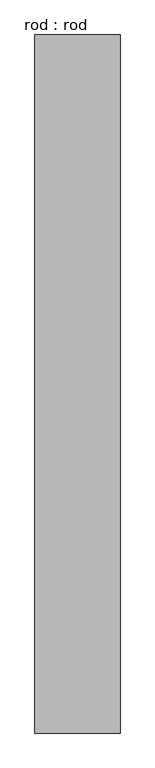
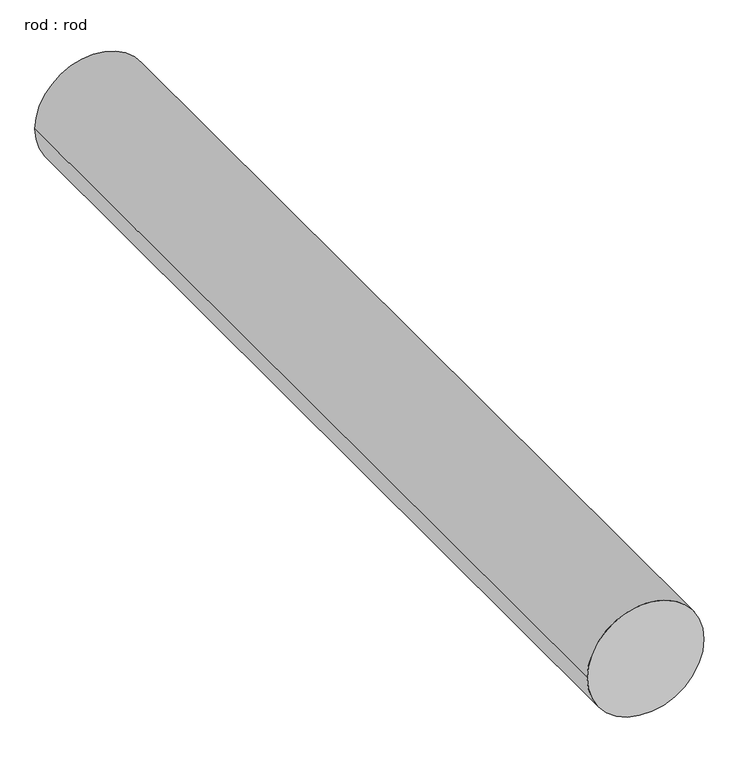
"""IFC4 building model written with IfcOpenShell, lengths in millimetres: proxy geometry, rod : rod."""

from ifc_helpers import new_model, si_unit, point, frame, frame_2d, origin, place, context, project, spatial, circle_curve, trimmed, segment, composite_curve, outline, extrude, source, transform, mapped, element, save


def rod_rod_53ca1b52(model_context):
    return source(origin(), model_context, "Body", "SweptSolid", [
        extrude(outline(composite_curve([segment(trimmed(circle_curve(frame_2d((0.0108462, 0.0)), 200.0), [point((0.0108462, 200.0))], [point((0.0108462, -200.0))], False, "CARTESIAN"), True, "CONTINUOUS"), segment(trimmed(circle_curve(frame_2d((0.0108462, 0.0)), 200.0), [point((0.0108462, -200.0))], [point((0.0108462, 200.0))], False, "CARTESIAN"), True, "CONTINUOUS")], self_intersect=False)), frame((0.0, 2452.7286153, 0.0), z_axis=(0.0, 1.0, 0.0), x_axis=(0.0, 0.0, 1.0)), (0.0, 0.0, 1.0), 3280.0),
    ])


if __name__ == "__main__":
    model = new_model("IFC4")
    model_context = context("Model", 3, world=origin())
    ifc_project = project(units=[si_unit("LENGTHUNIT", "METRE", prefix="MILLI")], contexts=[model_context])
    site = spatial("IfcSite", under=ifc_project)
    building = spatial("IfcBuilding", under=site)
    placement = place(None, origin())
    rod_rod_shape = rod_rod_53ca1b52(model_context)
    element("IfcBuildingElementProxy", 1, Name="rod : rod", ObjectType="rod : rod", at=placement, inside=building, context=model_context, shape_type="MappedRepresentation", body=[
        mapped(rod_rod_shape, transform((0.0, 0.0, 0.0), x_axis=(1.0, 0.0, 0.0), y_axis=(0.0, 1.0, 0.0), z_axis=(0.0, 0.0, 1.0))),
    ])
    save(model, "model.ifc")

# Revit data of these elements
# Type "rod : rod"
#   Default Elevation = 0
